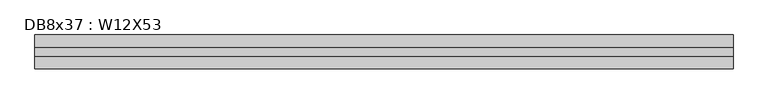
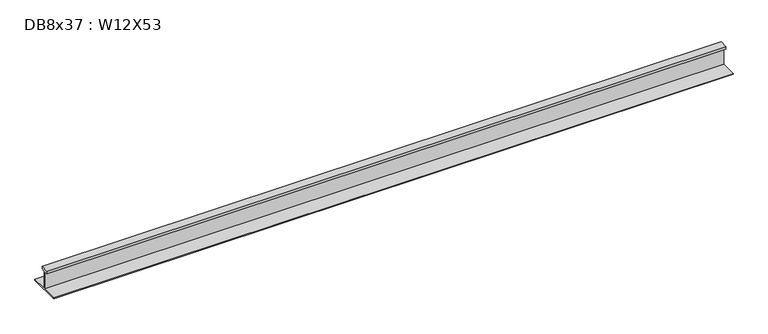
"""IFC4 building model written with IfcOpenShell, lengths in millimetres: beam geometry, DB8x37 : W12X53."""

from ifc_helpers import new_model, si_unit, frame, origin, place, context, project, spatial, polyline, outline, extrude, source, transform, mapped, element, save


def db8x37_w12x53_4562b796(model_context):
    return source(origin(), model_context, "Body", "SweptSolid", [
        extrude(outline(polyline([(38.1, 145.415), (38.1, 120.015), (2.921, 120.015), (2.921, -48.4505), (152.4, -48.4505), (152.4, -58.1025), (-152.4, -58.1025), (-152.4, -48.4505), (-2.921, -48.4505), (-2.921, 120.015), (-38.1, 120.015), (-38.1, 145.415), (38.1, 145.415)])), frame((-3138.17, 0.0, 0.0), z_axis=(1.0, 0.0, 0.0), x_axis=(0.0, 1.0, 0.0)), (0.0, 0.0, 1.0), 6303.899),
    ])


if __name__ == "__main__":
    model = new_model("IFC4")
    model_context = context("Model", 3, world=origin())
    ifc_project = project(units=[si_unit("LENGTHUNIT", "METRE", prefix="MILLI")], contexts=[model_context])
    site = spatial("IfcSite", under=ifc_project)
    building = spatial("IfcBuilding", under=site)
    placement = place(None, origin())
    db8x37_w12x53_shape = db8x37_w12x53_4562b796(model_context)
    element("IfcBeam", 1, ObjectType="DB8x37 : W12X53", at=placement, inside=building, context=model_context, shape_type="MappedRepresentation", body=[
        mapped(db8x37_w12x53_shape, transform((0.0, 0.0, 0.0), x_axis=(1.0, 0.0, 0.0), y_axis=(0.0, 1.0, 0.0), z_axis=(0.0, 0.0, 1.0))),
    ])
    save(model, "model.ifc")

# Revit data of these elements
# Type "DB8x37 : W12X53"
#   Assembly Code = "B10"
#   W = 53
#   Length [instance default] = 5' - 0"
#   bf = 0' - 10"
#   d = 1' - 0.1"
#   k = 0' - 1 3/8"
#   k2 = 0' - 0.8"
#   tf = 0' - 0.575"
#   tw = 0' - 0.345"
#   A = 0.108333 SF
#   Structural Material [instance default] = Steel ASTM A992
# Element 1 (IfcBeam, "DB8x37 : W12X53")
#   Materials on its faces: "Steel ASTM A992"
# Materials
#   "Steel ASTM A992": class "Metal", colour RGB 199 199 199, transparency 0, Description = "Structural steel 50ksi", Cost = 0
